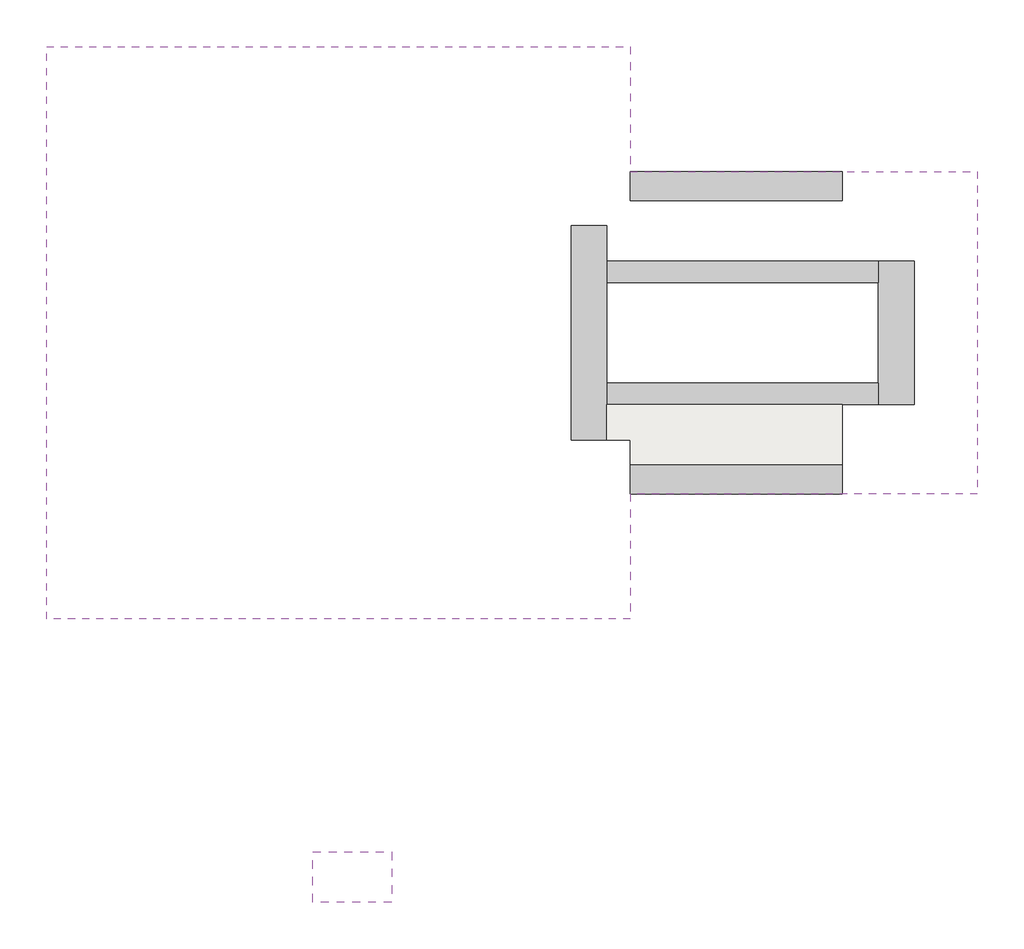
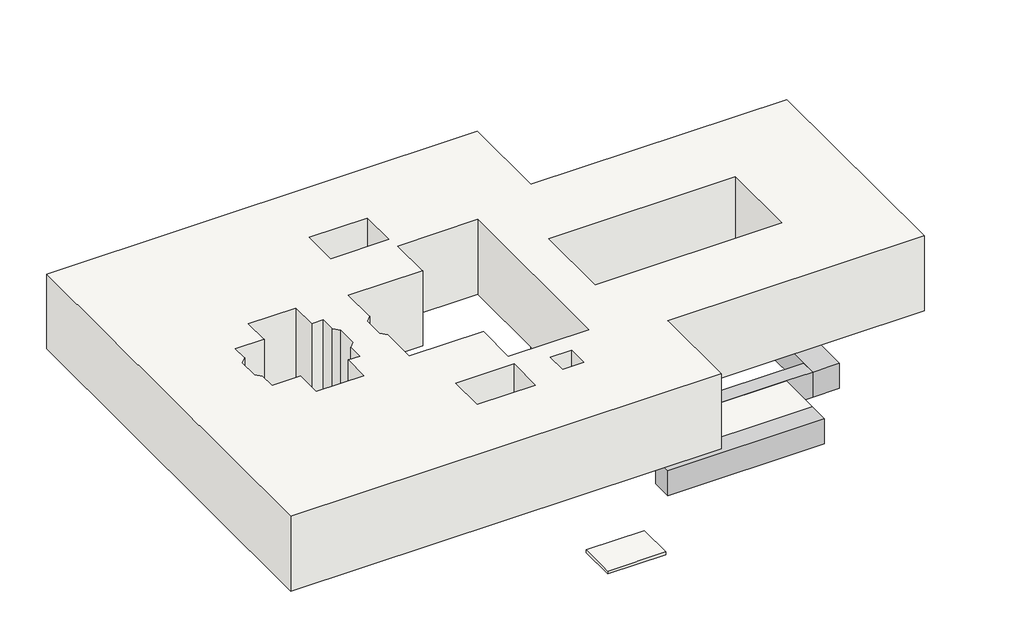
# One storey: 6 beams, 3 slabs.
"""IFC4 building model written with IfcOpenShell, lengths in millimetres."""

from ifc_helpers import new_model, si_unit, frame, origin, place, context, project, spatial, polyline, outline, extrude, faceted_brep, element, save

model = new_model("IFC4")

# Units and contexts
model_context = context("Model", 3, world=origin())
ifc_project = project(units=[si_unit("LENGTHUNIT", "METRE", prefix="MILLI")], contexts=[model_context])

# Site, building, storey
site = spatial("IfcSite", under=ifc_project)
building = spatial("IfcBuilding", under=site)
storey = spatial("IfcBuildingStorey", under=building, Name="T.O.C(MEZZ)", Elevation=7000.0)

# Beams
placement = place(None, origin())
element("IfcBeam", 1, ObjectType="Concrete-Rectangular-Beam : BM111_1000x1000_MG1", at=placement, inside=storey, context=model_context, shape_type="Brep", body=[
    faceted_brep([(15650.0, 8999.5208589, 7000.0), (16650.0, 8999.5208589, 7000.0), (16650.0, 9999.5208589, 7000.0), (16650.0, 10599.5208589, 7000.0), (16650.0, 13399.5208589, 7000.0), (16650.0, 13999.5208589, 7000.0), (16650.0, 14999.5208589, 7000.0), (15650.0, 14999.5208589, 7000.0), (15650.0, 8999.5208589, 6000.0), (15650.0, 14999.5208589, 6000.0), (16650.0, 8999.5208589, 6000.0), (16650.0, 14999.5208589, 6000.0), (16650.0, 13999.5208589, 6000.0), (16650.0, 13399.5208589, 6000.0), (16650.0, 10599.5208589, 6000.0), (16650.0, 9999.5208589, 6000.0), (16650.0, 8999.5208589, 6500.0)], [[[0, 1, 2, 3, 4, 5, 6, 7]], [[8, 0, 7, 9]], [[10, 8, 9, 11, 12, 13, 14, 15]], [[1, 16, 10, 15, 14, 13, 12, 11, 6, 5, 4, 3, 2]], [[1, 0, 8, 10, 16]], [[6, 11, 9, 7]]]),
])
element("IfcBeam", 2, ObjectType="Concrete-Rectangular-Beam : BM111_1000x1000_MG1", at=placement, inside=storey, context=model_context, shape_type="Brep", body=[
    faceted_brep([(24230.0, 9999.5208589, 7000.0), (25230.0, 9999.5208589, 7000.0), (25230.0, 13999.5208589, 7000.0), (24230.0, 13999.5208589, 7000.0), (24230.0, 13399.5208589, 7000.0), (24230.0, 10599.5208589, 7000.0), (24230.0, 9999.5208589, 6000.0), (24230.0, 13999.5208589, 6000.0), (24230.0, 13399.5208589, 6000.0), (24230.0, 10599.5208589, 6000.0), (25230.0, 9999.5208589, 6000.0), (25230.0, 13999.5208589, 6000.0)], [[[0, 1, 2, 3, 4, 5]], [[6, 0, 5, 4, 3, 7, 8, 9]], [[10, 6, 9, 8, 7, 11]], [[1, 10, 11, 2]], [[1, 0, 6, 10]], [[3, 2, 11, 7]]]),
])
element("IfcBeam", 3, ObjectType="Concrete-Rectangular-Beam : BM111_600x1000_MB1", at=placement, inside=storey, context=model_context, shape_type="Brep", body=[
    faceted_brep([(24230.0, 9999.5208589, 7000.0), (24230.0, 10599.5208589, 7000.0), (16650.0, 10599.5208589, 7000.0), (16650.0, 9999.5208589, 7000.0), (23229.9642165, 9999.5208589, 7000.0), (24230.0, 9999.5208589, 6000.0), (16650.0, 9999.5208589, 6500.0), (16650.0, 9999.5208589, 6000.0), (24230.0, 10599.5208589, 6000.0), (16650.0, 10599.5208589, 6000.0)], [[[0, 1, 2, 3, 4]], [[5, 0, 4, 3, 6, 7]], [[8, 5, 7, 9]], [[1, 8, 9, 2]], [[1, 0, 5, 8]], [[3, 2, 9, 7, 6]]]),
])
element("IfcBeam", 4, ObjectType="Concrete-Rectangular-Beam : BM111_600x1000_MB1", at=placement, inside=storey, context=model_context, shape_type="SweptSolid", body=[
    extrude(outline(polyline([(24230.0, 13999.5208589), (24230.0, 13399.5208589), (16650.0, 13399.5208589), (16650.0, 13999.5208589), (24230.0, 13999.5208589)])), frame((0.0, 0.0, 6000.0), z_axis=(0.0, 0.0, 1.0), x_axis=(1.0, 0.0, 0.0)), (0.0, 0.0, 1.0), 1000.0),
])
element("IfcBeam", 5, ObjectType="Concrete-Rectangular-Beam : BM111_800x1000_MG2", at=placement, inside=storey, context=model_context, shape_type="Brep", body=[
    faceted_brep([(23229.9642165, 7499.5208589, 7000.0), (23229.9642165, 8299.5208589, 7000.0), (17299.9642165, 8299.5208589, 7000.0), (17299.9642165, 7499.5208589, 7000.0), (23229.9642165, 7499.5208589, 6000.0), (17299.9642165, 7499.5208589, 6000.0), (23229.9642165, 8299.5208589, 6000.0), (17299.9642165, 8299.5208589, 6000.0), (23229.9642165, 8299.5208589, 6500.0)], [[[0, 1, 2, 3]], [[4, 0, 3, 5]], [[6, 4, 5, 7]], [[1, 8, 6, 7, 2]], [[2, 7, 5, 3]], [[1, 0, 4, 6, 8]]]),
])
element("IfcBeam", 6, ObjectType="Concrete-Rectangular-Beam : BM111_800x1000_MG2", at=placement, inside=storey, context=model_context, shape_type="SweptSolid", body=[
    extrude(outline(polyline([(23230.0, 16499.5208589), (23230.0, 15699.5208589), (17300.0, 15699.5208589), (17300.0, 16499.5208589), (23230.0, 16499.5208589)])), frame((0.0, 0.0, 6000.0), z_axis=(0.0, 0.0, 1.0), x_axis=(1.0, 0.0, 0.0)), (0.0, 0.0, 1.0), 1000.0),
])

# Slabs
element("IfcSlab", 7, ObjectType="CFS11_ROOF WATERPROOFING SYSTEM)", at=placement, inside=storey, context=model_context, shape_type="SweptSolid", body=[
    extrude(outline(polyline([(10638.4707406, -2508.5897214), (10638.4707406, -3908.5897214), (8438.4707406, -3908.5897214), (8438.4707406, -2508.5897214), (10638.4707406, -2508.5897214)])), frame((0.0, 0.0, 12890.0), z_axis=(0.0, 0.0, 1.0), x_axis=(1.0, 0.0, 0.0)), (0.0, 0.0, 1.0), 110.0),
])
element("IfcSlab", 8, ObjectType="MF00_3000", at=placement, inside=storey, context=model_context, shape_type="SweptSolid", body=[
    extrude(outline(polyline([(17299.9642165, 19999.5208589), (17299.9642165, 16499.5208589), (26999.9642165, 16499.5208589), (26999.9642165, 7499.5208589), (17299.9642165, 7499.5208589), (17299.9642165, 3999.5208589), (999.9642165, 3999.5208589), (999.9642165, 19999.5208589), (17299.9642165, 19999.5208589)]), holes=[polyline([(23333.9642165, 13519.5208589), (16273.9642165, 13519.5208589), (16273.9642165, 10479.5208589), (23333.9642165, 10479.5208589), (23333.9642165, 13519.5208589)]), polyline([(9504.9642165, 17509.5208589), (9504.9642165, 16109.5208589), (11704.9642165, 16109.5208589), (11704.9642165, 17509.5208589), (9504.9642165, 17509.5208589)]), polyline([(9504.9642165, 7889.5208589), (9504.9642165, 6489.5208589), (11704.9642165, 6489.5208589), (11704.9642165, 7889.5208589), (9504.9642165, 7889.5208589)]), polyline([(13725.9642165, 7619.5208589), (12925.9642165, 7619.5208589), (12925.9642165, 6819.5208589), (13725.9642165, 6819.5208589), (13725.9642165, 7619.5208589)]), polyline([(11769.9642165, 13999.5208589), (8962.9642165, 13999.5208589), (8962.9642165, 12599.5208589), (8762.9642165, 12399.5208589), (8762.9642165, 11599.5208589), (8962.9642165, 11399.5208589), (8962.9642165, 9999.5208589), (11769.9642165, 9999.5208589), (11769.9642165, 8369.5208589), (14799.9642165, 8369.5208589), (14799.9642165, 15629.5208589), (11769.9642165, 15629.5208589), (11769.9642165, 13999.5208589)]), polyline([(5307.9642165, 14229.5208589), (5307.9642165, 13199.5208589), (4222.9642165, 13199.5208589), (4222.9642165, 12599.5208589), (4022.9642165, 12399.5208589), (4022.9642165, 11599.5208589), (4222.9642165, 11399.5208589), (4222.9642165, 10799.5208589), (5307.9642165, 10799.5208589), (5307.9642165, 9769.5208589), (7107.9642165, 9769.5208589), (7107.9642165, 10799.5208589), (7542.9642165, 10799.5208589), (7542.9642165, 11399.5208589), (7742.9642165, 11599.5208589), (7742.9642165, 12399.5208589), (7542.9642165, 12599.5208589), (7542.9642165, 13199.5208589), (7107.9642165, 13199.5208589), (7107.9642165, 14229.5208589), (5307.9642165, 14229.5208589)])]), frame((0.0, 0.0, 10000.0), z_axis=(0.0, 0.0, 1.0), x_axis=(1.0, 0.0, 0.0)), (0.0, 0.0, 1.0), 3000.0),
])
element("IfcSlab", 9, ObjectType="MS1_200", at=placement, inside=storey, context=model_context, shape_type="SweptSolid", body=[
    extrude(outline(polyline([(16650.0, 8999.5208589), (16650.0, 9999.5208589), (23229.9642165, 9999.5208589), (23229.9642165, 8299.5208589), (17300.0, 8299.5208589), (17300.0, 8999.5208589), (16650.0, 8999.5208589)])), frame((0.0, 0.0, 6500.0), z_axis=(0.0, 0.0, 1.0), x_axis=(1.0, 0.0, 0.0)), (0.0, 0.0, 1.0), 500.0),
])

save(model, "model.ifc")

# Revit data of these elements
# Type "Concrete-Rectangular-Beam : BM111_1000x1000_MG1"
#   중앙부 하부근 = ""
#   중앙부 상부근 = ""
#   중앙부 보조근 = ""
#   중앙부 늑근 = ""
#   외단부 하부근 = ""
#   외단부 상부근 = ""
#   외단부 보조근 = ""
#   외단부 늑근 = ""
#   부호 = ""
#   내단부 하부근 = ""
#   내단부 상부근 = ""
#   내단부 보조근 = ""
#   내단부 늑근 = ""
#   ALL 하부근 = ""
#   ALL 상부근 = ""
#   ALL 보조근 = ""
#   ALL 늑근 = ""
#   Width = 1000 mm
#   Height = 1000 mm
#   Length [instance default] = 1524 mm
#   b = 1000 mm
#   h = 1000 mm
#   Structural Material [instance default] = 콘크리트 - 현장타설 콘크리트
#   hec_material3 [instance default] = none
#   hec_material2 [instance default] = none
#   hec_material1 [instance default] = none
#   Assembly Code = ""
# Type "Concrete-Rectangular-Beam : BM111_600x1000_MB1"
#   중앙부 하부근 = ""
#   중앙부 상부근 = ""
#   중앙부 보조근 = ""
#   중앙부 늑근 = ""
#   외단부 하부근 = ""
#   외단부 상부근 = ""
#   외단부 보조근 = ""
#   외단부 늑근 = ""
#   부호 = ""
#   내단부 하부근 = ""
#   내단부 상부근 = ""
#   내단부 보조근 = ""
#   내단부 늑근 = ""
#   ALL 하부근 = ""
#   ALL 상부근 = ""
#   ALL 보조근 = ""
#   ALL 늑근 = ""
#   Width = 600 mm
#   Height = 1000 mm
#   Length [instance default] = 1524 mm
#   b = 600 mm
#   h = 1000 mm
#   Structural Material [instance default] = 콘크리트 - 현장타설 콘크리트
#   hec_material3 [instance default] = none
#   hec_material2 [instance default] = none
#   hec_material1 [instance default] = none
#   Assembly Code = ""
# Type "Concrete-Rectangular-Beam : BM111_800x1000_MG2"
#   중앙부 하부근 = ""
#   중앙부 상부근 = ""
#   중앙부 보조근 = ""
#   중앙부 늑근 = ""
#   외단부 하부근 = ""
#   외단부 상부근 = ""
#   외단부 보조근 = ""
#   외단부 늑근 = ""
#   부호 = ""
#   내단부 하부근 = ""
#   내단부 상부근 = ""
#   내단부 보조근 = ""
#   내단부 늑근 = ""
#   ALL 하부근 = ""
#   ALL 상부근 = ""
#   ALL 보조근 = ""
#   ALL 늑근 = ""
#   Width = 800 mm
#   Height = 1000 mm
#   Length [instance default] = 1524 mm
#   b = 800 mm
#   h = 1000 mm
#   Structural Material [instance default] = 콘크리트 - 현장타설 콘크리트
#   hec_material3 [instance default] = none
#   hec_material2 [instance default] = none
#   hec_material1 [instance default] = none
#   Assembly Code = ""
# Type "CFS11_ROOF WATERPROOFING SYSTEM)"
#   Keynote = ""
#   Type Comments = "구조_콘크리트"
#   Function = 0
#   Layers, outside or top first: 60 mm "A04AP089-00001_Protective Concrete w/ Steel Trowel Finish" (function 4); 50 mm "22212-220641_Roof Insulation_thk50" (function 3); 0 mm "A04AP012-00001_PE Sheet (Vapor Barrier)_Roof" (function 100); 0 mm "A04AP000-00001_Roof_Waterproofing Membrane" (function 100)
# Type "MF00_3000"
#   Type Comments = "구조_콘크리트"
#   Layers, outside or top first: 3000 mm "14200-030101_Concrete Pouring" (function 1)
# Type "MS1_200"
#   Type Comments = "구조_콘크리트"
#   Layers, outside or top first: 500 mm "콘크리트" (function 1)
# Elements 1, 2 (IfcBeam, "Concrete-Rectangular-Beam : BM111_1000x1000_MG1")
#   Comments = ""
#   Structural Material = 콘크리트 - 현장타설 콘크리트
#   hec_material3 = none
#   hec_material2 = none
#   hec_material1 = none
#   Phase Created = New Construction
#   Materials on its faces: "콘크리트 - 현장타설 콘크리트"
# Elements 3, 4 (IfcBeam, "Concrete-Rectangular-Beam : BM111_600x1000_MB1")
#   Comments = ""
#   Structural Material = 콘크리트 - 현장타설 콘크리트
#   hec_material3 = none
#   hec_material2 = none
#   hec_material1 = none
#   Phase Created = New Construction
#   Materials on its faces: "콘크리트 - 현장타설 콘크리트"
# Elements 5, 6 (IfcBeam, "Concrete-Rectangular-Beam : BM111_800x1000_MG2")
#   Comments = ""
#   Structural Material = 콘크리트 - 현장타설 콘크리트
#   hec_material3 = none
#   hec_material2 = none
#   hec_material1 = none
#   Phase Created = New Construction
#   Materials on its faces: "콘크리트 - 현장타설 콘크리트"
# Element 7 (IfcSlab, "CFS11_ROOF WATERPROOFING SYSTEM)")
#   Comments = ""
#   TMP_Element Name = "SS2"
#   built-in parameter 1001955 = 1.5708 (stored number, unit not read)
#   Height Offset From Level = 0 mm
#   built-in parameter 1001954 = 1
#   Phase Created = New Construction
#   Materials on its faces: "A04AP000-00001_Roof_Waterproofing Membrane", "A04AP089-00001_Protective Concrete w/ Steel Trowel Finish"
# Element 8 (IfcSlab, "MF00_3000")
#   Comments = ""
#   Height Offset From Level = 0 mm
#   built-in parameter 1001954 = 1
#   Phase Created = New Construction
#   Materials on its faces: "14200-030101_Concrete Pouring"
# Element 9 (IfcSlab, "MS1_200")
#   Comments = ""
#   built-in parameter 1001955 = -1.5708 (stored number, unit not read)
#   Height Offset From Level = 0 mm
#   built-in parameter 1001954 = 1
#   Phase Created = New Construction
#   Materials on its faces: "콘크리트"
# Materials
#   "콘크리트 - 현장타설 콘크리트": class "콘크리트", colour RGB 192 192 192, transparency 0
#   "A04AP089-00001_Protective Concrete w/ Steel Trowel Finish": class "Concrete", colour RGB 176 176 176, transparency 0, Description = "Plain Conc.", W00) Work Master Code = "A04AP089-00001", W01) Work Master_Lv1 = "Finishing Work", W02) Work Master_Lv2 = "Roof Work", W03) Work Master_Spec.1 = "Protective Concrete w/ Steel Trowel Finish", Cost = 0
#   "22212-220641_Roof Insulation_thk50": class "Insulation", colour RGB 255 255 217, transparency 0, Description = "Insulation(Rigid)", W00) Work Master Code = "22212-220641", W01) Work Master_Lv1 = "Finishing Work", W02) Work Master_Lv2 = "Roof Work", W03) Work Master_Spec.1 = "Roof Insulation", W04) Work Master_Spec.2 = "Rigid Extruded Polystyrene Foam Insulation", W05) Work Master_Spec.3 = "THK=50mm", Cost = 0
#   "A04AP012-00001_PE Sheet (Vapor Barrier)_Roof": class "Finish", colour RGB 128 128 64, transparency 0, Description = "Plastic", W00) Work Master Code = "A04AP012-00001", W01) Work Master_Lv1 = "Finishing Work", W02) Work Master_Lv2 = "Roof Work", W03) Work Master_Spec.1 = "PE Sheet (Vapor Barrier)", Cost = 0
#   "A04AP000-00001_Roof_Waterproofing Membrane": class "Plastic", colour RGB 127 127 127, transparency 0, Description = "Exterior finish, roofing", W00) Work Master Code = "A04AP000-00001", W01) Work Master_Lv1 = "Finishing Work", W02) Work Master_Lv2 = "Roof Work", W03) Work Master_Spec.1 = "Waterproofing Membrane", W04) Work Master_Spec.2 = "EPDM(or Equivalent)", W05) Work Master_Spec.3 = "w/ Accessories", Cost = 0
#   "14200-030101_Concrete Pouring": class "Concrete", colour RGB 176 176 176, transparency 0, Description = "Reinf. Conc.", W00) Work Master Code = "14200-030101", W01) Work Master_Lv1 = "Concrete Work", W02) Work Master_Lv2 = "Building/Shelter Foundation Work", W03) Work Master_Spec.1 = "Concrete Pouring", W04) Work Master_Spec.2 = "F'c (Cylinder Strength) > 35MPa", W05) Work Master_Spec.3 = "Cement Type-1", Cost = 0
#   "콘크리트": class "*D 철근콘크리트공사", colour RGB 192 192 192, transparency 0, Keynote = "DF", Description = "콘크리트", Cost = 0
# Room, not placed, phase "New Construction", upper offset 0 mm, lower offset 0 mm
#   Comments = ""
#   Number = "19"
#   Name = ""
#   S01) Room Name = ""
#   S02) Room Number(Project) = ""
# Room, not placed, phase "New Construction", upper offset 0 mm, lower offset 0 mm
#   Comments = ""
#   Number = "128"
#   Name = ""
# Room, not placed, phase "New Construction", upper offset 0 mm, lower offset 0 mm
#   Comments = ""
#   Base Finish = "EXPOXY PAINT ON THK.15 CEMENT PLASTER(H=100)"
#   Ceiling Finish = "LATEX PAINT ON FAIR FACED CONC."
#   Wall Finish = "H=1.5M ACID RESISTANT PAINT ON THK.15 CEMENT PLASTER ABOVE 1.5M LATEXT PAINT ON THK. 15 CEMENT PLASTER"
#   Floor Finish = "ACID RESISTANT PAINT ON STEEL TROWELED CONC' SLAB"
#   Number = ""
#   Name = ""
#   F01) Building Name = "CENTRAL CONTROL BUILDING"
#   S01) Room Name = "BATTERY ROOM"
#   S02) Room Number(Project) = "UCA02R0002"
# Room, not placed, phase "New Construction", upper offset 0 mm, lower offset 0 mm
#   Comments = ""
#   Base Finish = "EXPOXY PAINT ON THK.15 CEMENT PLASTER(H=100)"
#   Ceiling Finish = "LATEX PAINT ON FAIR FACED CONC."
#   Wall Finish = "LATEX PAINT ON THK.15 CEMENT PLASTER + MASONRY WALL"
#   Floor Finish = "EPOXY PAINT ON STEEL TROWELED CONC. SLAB"
#   Number = ""
#   Name = ""
#   F01) Building Name = "CENTRAL CONTROL BUILDING"
#   S01) Room Name = "SWITCHGEAR ROOM"
#   S02) Room Number(Project) = "UCA02R0001"
# Room, not placed, phase "New Construction", upper offset 0 mm, lower offset 0 mm
#   Comments = ""
#   Base Finish = "EXPOXY PAINT ON THK.15 CEMENT PLASTER(H=100)"
#   Ceiling Finish = "LATEX PAINT ON FAIR FACED CONC."
#   Wall Finish = "LATEX PAINT ON THK.15 CEMENT PLASTER + MASONRY WALL"
#   Floor Finish = "EPOXY PAINT ON STEEL TROWELED CONC. SLAB"
#   Number = ""
#   Name = ""
#   F01) Building Name = "CENTRAL CONTROL BUILDING"
#   S01) Room Name = "ELECTRONIC ROOM"
#   S02) Room Number(Project) = "UCA03R0001"
# Room, not placed, phase "New Construction", upper offset 0 mm, lower offset 0 mm
#   Comments = ""
#   Base Finish = "EXPOXY PAINT ON THK.15 CEMENT PLASTER(H=100)"
#   Ceiling Finish = "LATEX PAINT ON FAIR FACED CONC."
#   Wall Finish = "LATEX PAINT ON THK.15 CEMENT PLASTER + MASONRY WALL"
#   Floor Finish = "EPOXY PAINT ON STEEL TROWELED CONC. SLAB"
#   Number = ""
#   Name = ""
#   F01) Building Name = "CENTRAL CONTROL BUILDING"
#   S01) Room Name = "ELECTRICAL ROOM"
#   S02) Room Number(Project) = "UCA03R0002"
# Room, not placed, phase "New Construction", upper offset 0 mm, lower offset 0 mm
#   Comments = ""
#   Base Finish = "RUBBER BASE(H=100)"
#   Ceiling Finish = "SUSPENDED MINERAL FIBERBOARD PANEL(GRID 600x600)"
#   Wall Finish = "LATEX PAINT ON THK.15 CEMENT PLASTER + MASONRY WALL"
#   Floor Finish = "PVC TILE W/ADHESIVE ON STEEL TROWELED CONC. SLAB"
#   Number = ""
#   Name = ""
#   F01) Building Name = "CENTRAL CONTROL BUILDING"
#   S01) Room Name = "CORRIDOR"
#   S02) Room Number(Project) = "UCA03R0003"
# Room, not placed, phase "New Construction", upper offset 0 mm, lower offset 0 mm
#   Comments = ""
#   Base Finish = "RUBBER BASE(H=100)"
#   Ceiling Finish = "LATEX PAINT ON FAIR FACED CONC."
#   Wall Finish = "LATEX PAINT ON THK.15 CEMENT PLASTER + MASONRY WALL"
#   Floor Finish = "PVC TILE W/ADHESIVE ON STEEL TROWELED CONC. SLAB"
#   Number = ""
#   Name = ""
#   F01) Building Name = "CENTRAL CONTROL BUILDING"
#   S01) Room Name = "STAIRWAY"
#   S02) Room Number(Project) = "UCA03R0004"
# Room, not placed, phase "New Construction", upper offset 0 mm, lower offset 0 mm
#   Comments = ""
#   Base Finish = "RUBBER BASE(H=100)"
#   Ceiling Finish = "LATEX PAINT ON FAIR FACED CONC."
#   Wall Finish = "LATEX PAINT ON THK.15 CEMENT PLASTER + MASONRY WALL"
#   Floor Finish = "PVC TILE W/ADHESIVE ON STEEL TROWELED CONC. SLAB"
#   Number = ""
#   Name = ""
#   F01) Building Name = "CENTRAL CONTROL BUILDING"
#   S01) Room Name = "STAIRWAY"
#   S02) Room Number(Project) = "UCA02R0003"
